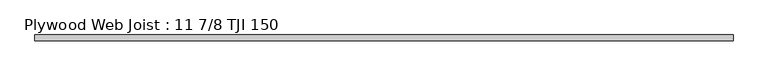
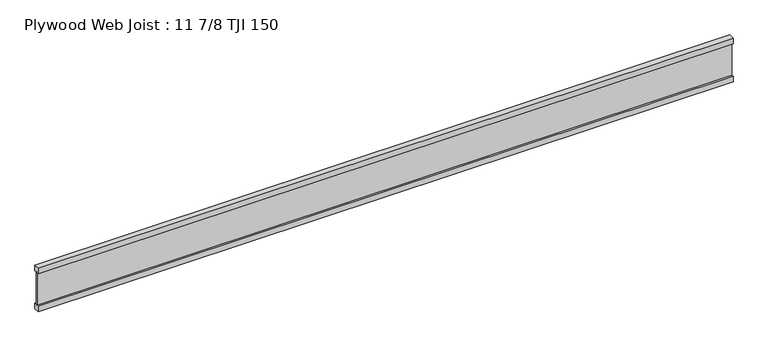
"""IFC4 building model written with IfcOpenShell, lengths in millimetres: beam geometry, Plywood Web Joist : 11 7/8 TJI 150."""

from ifc_helpers import new_model, si_unit, frame, origin, place, context, project, spatial, polyline, outline, extrude, source, transform, mapped, element, save


def plywood_web_joist_11_7_8_tji_150_914fbb7f(model_context):
    return source(origin(), model_context, "Body", "SweptSolid", [
        extrude(outline(polyline([(-19.05, 150.8125), (19.05, 150.8125), (19.05, 112.7125), (4.7625, 112.7125), (4.7625, 119.0625), (-4.7625, 119.0625), (-4.7625, 112.7125), (-19.05, 112.7125), (-19.05, 150.8125)])), frame((-2272.50625, 0.0, 0.0), z_axis=(1.0, 0.0, 0.0), x_axis=(0.0, 1.0, 0.0)), (0.0, 0.0, 1.0), 4545.0125),
        extrude(outline(polyline([(19.05, -112.7125), (19.05, -150.8125), (-19.05, -150.8125), (-19.05, -112.7125), (-4.7625, -112.7125), (-4.7625, -118.3285374), (4.7625, -118.3285374), (4.7625, -112.7125), (19.05, -112.7125)])), frame((-2272.50625, 0.0, 0.0), z_axis=(1.0, 0.0, 0.0), x_axis=(0.0, 1.0, 0.0)), (0.0, 0.0, 1.0), 4545.0125),
        extrude(outline(polyline([(2272.50625, 4.7625), (2272.50625, -4.7625), (-2272.50625, -4.7625), (-2272.50625, 4.7625), (2272.50625, 4.7625)])), frame((0.0, 0.0, -118.3285374), z_axis=(0.0, 0.0, 1.0), x_axis=(1.0, 0.0, 0.0)), (0.0, 0.0, 1.0), 237.3910374),
    ])


if __name__ == "__main__":
    model = new_model("IFC4")
    model_context = context("Model", 3, world=origin())
    ifc_project = project(units=[si_unit("LENGTHUNIT", "METRE", prefix="MILLI")], contexts=[model_context])
    site = spatial("IfcSite", under=ifc_project)
    building = spatial("IfcBuilding", under=site)
    placement = place(None, origin())
    plywood_web_joist_11_7_8_tji_150_shape = plywood_web_joist_11_7_8_tji_150_914fbb7f(model_context)
    element("IfcBeam", 1, ObjectType="Plywood Web Joist : 11 7/8 TJI 150", at=placement, inside=building, context=model_context, shape_type="MappedRepresentation", body=[
        mapped(plywood_web_joist_11_7_8_tji_150_shape, transform((0.0, 0.0, 0.0), x_axis=(1.0, 0.0, 0.0), y_axis=(0.0, 1.0, 0.0), z_axis=(0.0, 0.0, 1.0))),
    ])
    save(model, "model.ifc")

# Revit data of these elements
# Type "Plywood Web Joist : 11 7/8 TJI 150"
#   Assembly Code = "B10"
#   Cost = 17.5
#   Length [instance default] = 5' - 0"
#   b = 0' - 1 1/2"
#   d = 0' - 11 7/8"
#   Structural Material [instance default] = Softwood, Lumber
# Element 1 (IfcBeam, "Plywood Web Joist : 11 7/8 TJI 150")
#   Structural Material = Douglas Fir #2
#   Materials on its faces: "Douglas Fir #2"
# Materials
#   "Softwood, Lumber": class "Wood", colour RGB 223 192 134, transparency 0, Description = "Pinus Echinata", Cost = 0
#   "Douglas Fir #2": class "Wood", colour RGB 223 192 134, transparency 0, Description = "Pinus Echinata", Cost = 0
